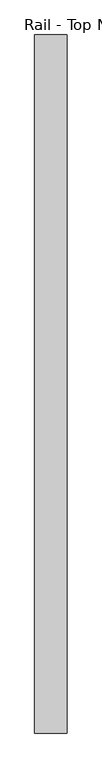
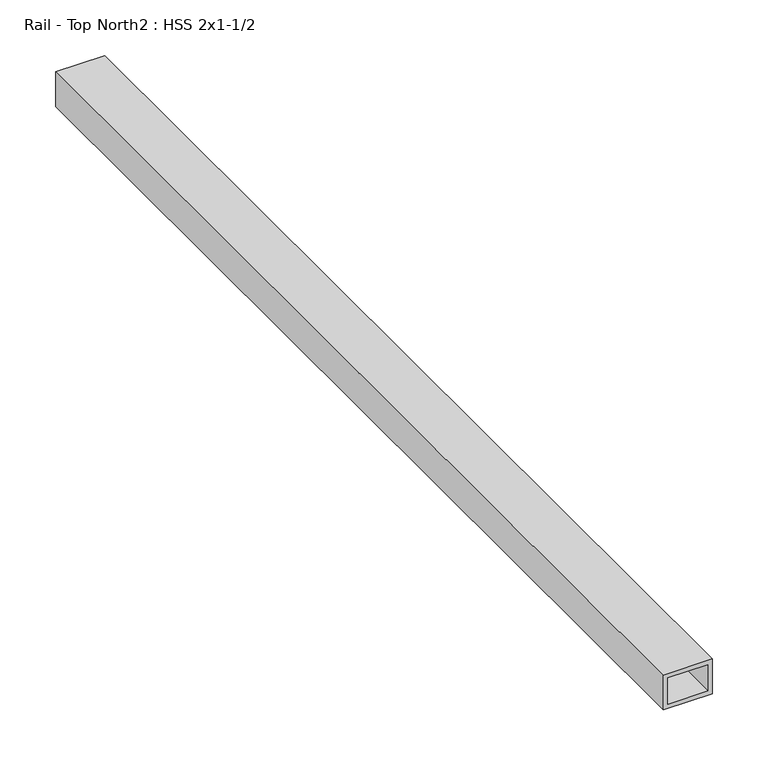
"""IFC4 building model written with IfcOpenShell, lengths in millimetres: proxy geometry, Rail - Top North2 : HSS 2x1-1/2."""

from ifc_helpers import new_model, si_unit, frame, origin, place, context, project, spatial, polyline, outline, extrude, source, transform, mapped, element, save


def rail_top_north2_hss_2x1_1_2_493d1250(model_context):
    return source(origin(), model_context, "Body", "SweptSolid", [
        extrude(outline(polyline([(2400.3, 587416.6934739), (2438.4, 587416.6934739), (2438.4, 587365.8934739), (2400.3, 587365.8934739), (2400.3, 587416.6934739)]), holes=[polyline([(2433.6375, 587411.9309739), (2405.0625, 587411.9309739), (2405.0625, 587370.6559739), (2433.6375, 587370.6559739), (2433.6375, 587411.9309739)])]), frame((0.0, -532877.4663841, 0.0), z_axis=(0.0, 1.0, 0.0), x_axis=(0.0, 0.0, 1.0)), (0.0, 0.0, 1.0), 1092.2),
    ])


if __name__ == "__main__":
    model = new_model("IFC4")
    model_context = context("Model", 3, world=origin())
    ifc_project = project(units=[si_unit("LENGTHUNIT", "METRE", prefix="MILLI")], contexts=[model_context])
    site = spatial("IfcSite", under=ifc_project)
    building = spatial("IfcBuilding", under=site)
    placement = place(None, origin())
    rail_top_north2_hss_2x1_1_2_shape = rail_top_north2_hss_2x1_1_2_493d1250(model_context)
    element("IfcBuildingElementProxy", 1, Name="Rail - Top North2 : HSS 2x1-1/2", ObjectType="Rail - Top North2 : HSS 2x1-1/2", at=placement, inside=building, context=model_context, shape_type="MappedRepresentation", body=[
        mapped(rail_top_north2_hss_2x1_1_2_shape, transform((0.0, 0.0, 0.0), x_axis=(1.0, 0.0, 0.0), y_axis=(0.0, 1.0, 0.0), z_axis=(0.0, 0.0, 1.0))),
    ])
    save(model, "model.ifc")

# Revit data of these elements
# Element 1 (IfcBuildingElementProxy, "Rail - Top North2 : HSS 2x1-1/2")
#   Materials on its faces: "1-1/2\"X2\" GALV. STL HSS TUBING"
# Materials
#   "1-1/2\"X2\" GALV. STL HSS TUBING": class "Generic", colour RGB 211 211 207, transparency 0, Cost = 0
